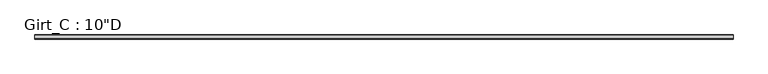
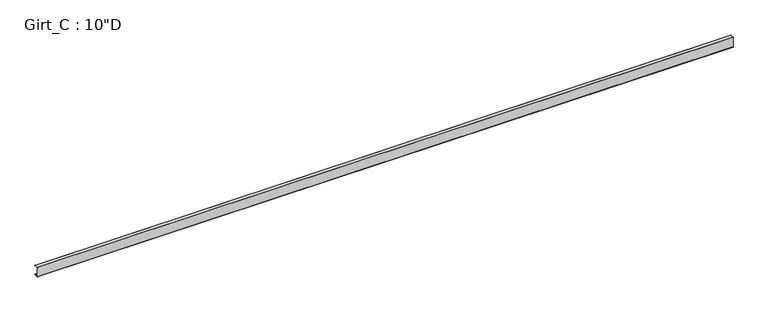
"""IFC4 building model written with IfcOpenShell, lengths in millimetres: beam geometry."""

from ifc_helpers import new_model, si_unit, point, frame, frame_2d, origin, place, context, project, spatial, polyline, circle_curve, trimmed, segment, composite_curve, outline, extrude, source, transform, mapped, element, save


def beam_473ee45a(model_context):
    return source(origin(), model_context, "Body", "SweptSolid", [
        extrude(outline(composite_curve([segment(polyline([(87.5109375, 127.0), (99.7560415, 112.4068534), (97.6278742, 110.621109), (86.2154765, 124.221875), (3.3005807, 124.221875)]), True, "CONTINUOUS"), segment(trimmed(circle_curve(frame_2d((3.3741066, 122.2381931)), 1.9850441), [point((3.3005807, 124.221875))], [point((1.3890625, 122.2381931))], True, "CARTESIAN"), True, "CONTINUOUS"), segment(polyline([(1.3890625, 122.2381931), (1.3890625, -122.2389339)]), True, "CONTINUOUS"), segment(trimmed(circle_curve(frame_2d((3.3748024, -122.2389339)), 1.9857399), [point((1.3890625, -122.2389339))], [point((3.2694106, -124.221875))], True, "CARTESIAN"), True, "CONTINUOUS"), segment(polyline([(3.2694106, -124.221875), (86.2154765, -124.221875), (97.6510975, -110.5934327), (99.7792647, -112.379177), (87.5109375, -127.0), (3.3734375, -127.0)]), True, "CONTINUOUS"), segment(trimmed(circle_curve(frame_2d((3.3734375, -122.2375)), 4.7625), [point((3.3734375, -127.0))], [point((-1.3890625, -122.2375))], False, "CARTESIAN"), True, "CONTINUOUS"), segment(polyline([(-1.3890625, -122.2375), (-1.3890625, 122.2375)]), True, "CONTINUOUS"), segment(trimmed(circle_curve(frame_2d((3.3734375, 122.2375)), 4.7625), [point((-1.3890625, 122.2375))], [point((3.3734375, 127.0))], False, "CARTESIAN"), True, "CONTINUOUS"), segment(polyline([(3.3734375, 127.0), (87.5109375, 127.0)]), True, "CONTINUOUS")], self_intersect=False)), frame((-8465.6549, 0.0, 0.0), z_axis=(1.0, 0.0, 0.0), x_axis=(0.0, 1.0, 0.0)), (0.0, 0.0, 1.0), 16928.338),
    ])


if __name__ == "__main__":
    model = new_model("IFC4")
    model_context = context("Model", 3, world=origin())
    ifc_project = project(units=[si_unit("LENGTHUNIT", "METRE", prefix="MILLI")], contexts=[model_context])
    site = spatial("IfcSite", under=ifc_project)
    building = spatial("IfcBuilding", under=site)
    placement = place(None, origin())
    beam_shape = beam_473ee45a(model_context)
    element("IfcBeam", 1, ObjectType="Girt_C : 10\"D", at=placement, inside=building, context=model_context, shape_type="MappedRepresentation", body=[
        mapped(beam_shape, transform((0.0, 0.0, 0.0), x_axis=(1.0, 0.0, 0.0), y_axis=(0.0, 1.0, 0.0), z_axis=(0.0, 0.0, 1.0))),
    ])
    save(model, "model.ifc")

# Revit data of these elements
# Type "Girt_C : 10\"D"
#   half leg = 0' - 1 3/4"
#   Web_Thickness = 0' - 0 7/64"
#   Length [instance default] = 10' - 0"
#   Leg_1 = 0' - 3 1/2"
#   Height = 0' - 10"
#   Structural Material [instance default] = none
